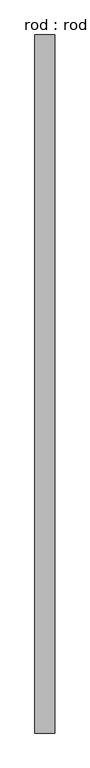
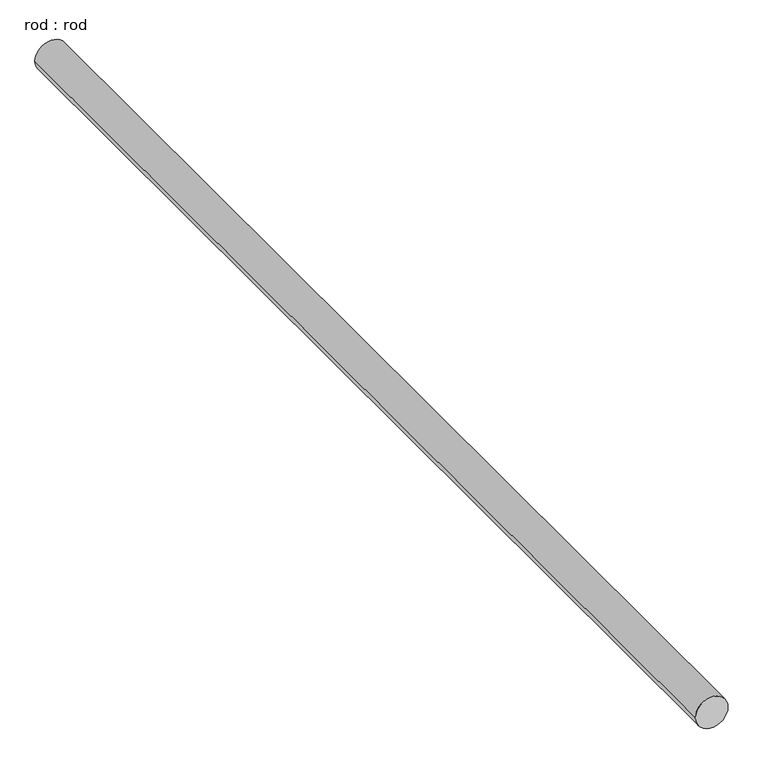
"""IFC4 building model written with IfcOpenShell, lengths in millimetres: proxy geometry, rod : rod."""

from ifc_helpers import new_model, si_unit, point, frame, frame_2d, origin, place, context, project, spatial, circle_curve, trimmed, segment, composite_curve, outline, extrude, source, transform, mapped, element, save


def rod_rod_faa0bf0a(model_context):
    return source(origin(), model_context, "Body", "SweptSolid", [
        extrude(outline(composite_curve([segment(trimmed(circle_curve(frame_2d((0.0108462, 0.0)), 200.0), [point((0.0108462, 200.0))], [point((0.0108462, -200.0))], False, "CARTESIAN"), True, "CONTINUOUS"), segment(trimmed(circle_curve(frame_2d((0.0108462, 0.0)), 200.0), [point((0.0108462, -200.0))], [point((0.0108462, 200.0))], False, "CARTESIAN"), True, "CONTINUOUS")], self_intersect=False)), frame((0.0, -2939.9255997, 0.0), z_axis=(0.0, 1.0, 0.0), x_axis=(0.0, 0.0, 1.0)), (0.0, 0.0, 1.0), 14065.3084301),
    ])


if __name__ == "__main__":
    model = new_model("IFC4")
    model_context = context("Model", 3, world=origin())
    ifc_project = project(units=[si_unit("LENGTHUNIT", "METRE", prefix="MILLI")], contexts=[model_context])
    site = spatial("IfcSite", under=ifc_project)
    building = spatial("IfcBuilding", under=site)
    placement = place(None, origin())
    rod_rod_shape = rod_rod_faa0bf0a(model_context)
    element("IfcBuildingElementProxy", 1, Name="rod : rod", ObjectType="rod : rod", at=placement, inside=building, context=model_context, shape_type="MappedRepresentation", body=[
        mapped(rod_rod_shape, transform((0.0, 0.0, 0.0), x_axis=(1.0, 0.0, 0.0), y_axis=(0.0, 1.0, 0.0), z_axis=(0.0, 0.0, 1.0))),
    ])
    save(model, "model.ifc")

# Revit data of these elements
# Type "rod : rod"
#   Default Elevation = 0
